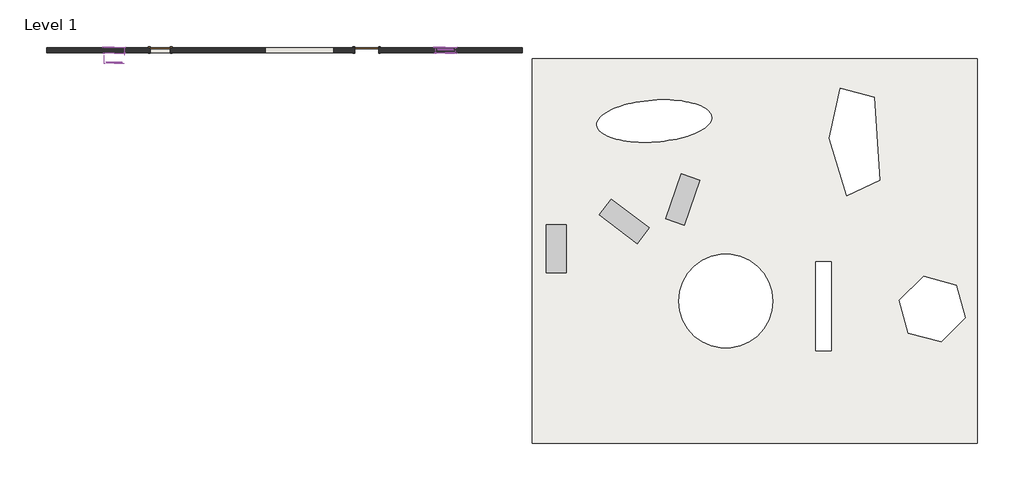
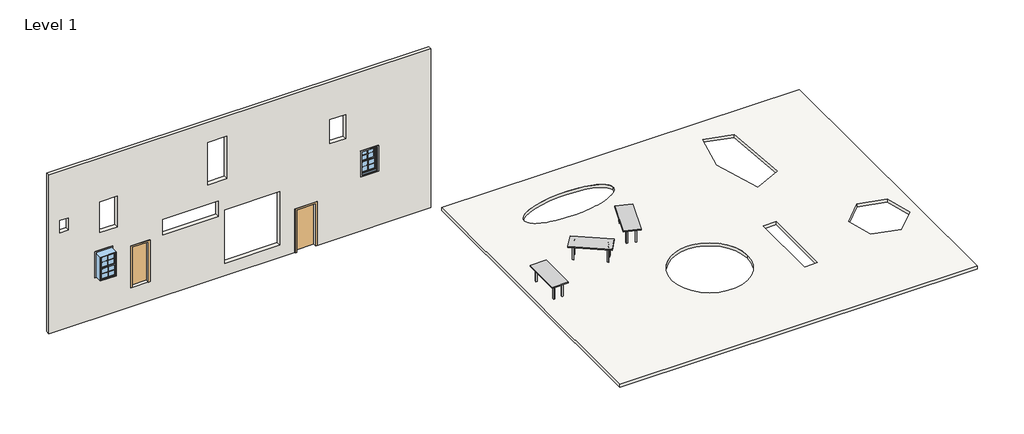
# One storey: 8 proxies, 3 furniture elements, 2 doors, 2 windows, 1 slab, 1 wall.
"""IFC4 building model written with IfcOpenShell, lengths in millimetres."""

import ifcopenshell
import ifcopenshell.guid

model = None  # the IFC model being written
_history = None  # IfcOwnerHistory: only IFC2X3 demands one
_inside = {}  # id of a spatial element -> (the spatial element, [elements in it])
_under = {}  # id of a project, library or spatial element -> (it, [spatial elements below it])
_declared = {}  # id of a project -> (the project, [libraries it declares])
_typed = {}  # id of a type object -> (the type object, [elements of that type])
_made_of = {}  # id of a material, layer set ... -> (it, [elements and type objects made of it])


def new_model(schema):
    """Start an empty IFC model of exactly this schema.

    Asked for "IFC4X3", IfcOpenShell would pick the latest addendum, in which some entities
    have other attributes; the version numbers below select the first issue.
    IFC2X3 requires an IfcOwnerHistory on every rooted entity: one is made here for all.
    """
    global model, _history
    if schema == "IFC4X3":
        model = ifcopenshell.file(schema_version=(4, 3, 0, 0))
    else:
        model = ifcopenshell.file(schema=schema)
    _inside.clear()
    _under.clear()
    _declared.clear()
    _typed.clear()
    _made_of.clear()
    _history = None
    if model.schema == "IFC2X3":
        org = make("IfcOrganization", Name="unknown")
        user = make(
            "IfcPersonAndOrganization",
            ThePerson=make("IfcPerson", FamilyName="unknown"),
            TheOrganization=org,
        )
        app = make(
            "IfcApplication",
            ApplicationDeveloper=org,
            Version="unknown",
            ApplicationFullName="unknown",
            ApplicationIdentifier="unknown",
        )
        _history = make(
            "IfcOwnerHistory",
            OwningUser=user,
            OwningApplication=app,
            ChangeAction="ADDED",
            CreationDate=0,
        )
    return model


def make(cls, **values):
    """One entity of the class cls with the attributes given. An attribute that is None is left unset."""
    return model.create_entity(
        cls, **{name: value for name, value in values.items() if value is not None}
    )


def rooted(cls, **values):
    """An entity with a GlobalId (a new one), such as an element, a storey or a relation."""
    return make(cls, GlobalId=ifcopenshell.guid.new(), OwnerHistory=_history, **values)


def si_unit(unit_type, name, prefix=None):
    """IfcSIUnit, for example si_unit("LENGTHUNIT", "METRE", prefix="MILLI")."""
    return make("IfcSIUnit", UnitType=unit_type, Prefix=prefix, Name=name)


def assignment(units):
    """IfcUnitAssignment: the units of a project."""
    return None if units is None else make("IfcUnitAssignment", Units=units)


def point(xyz):
    """IfcCartesianPoint."""
    return None if xyz is None else make("IfcCartesianPoint", Coordinates=xyz)


def direction(xyz):
    """IfcDirection."""
    return None if xyz is None else make("IfcDirection", DirectionRatios=xyz)


def frame(location, z_axis=None, x_axis=None):
    """IfcAxis2Placement3D, a coordinate frame: its origin and axes. An axis left out is left unset."""
    return make(
        "IfcAxis2Placement3D",
        Location=point(location),
        Axis=direction(z_axis),
        RefDirection=direction(x_axis),
    )


def origin():
    """The frame at (0, 0, 0) with its axes left unset."""
    return frame((0.0, 0.0, 0.0))


def origin_with_axes():
    """The frame at (0, 0, 0) with the z axis (0, 0, 1) and the x axis (1, 0, 0) written out."""
    return frame((0.0, 0.0, 0.0), z_axis=(0.0, 0.0, 1.0), x_axis=(1.0, 0.0, 0.0))


def place(relative_to, where):
    """IfcLocalPlacement: puts the frame where relative to a parent placement (None: the world)."""
    return make(
        "IfcLocalPlacement", PlacementRelTo=relative_to, RelativePlacement=where
    )


def context(
    kind, dimensions, precision=None, world=None, true_north=None, identifier=None
):
    """IfcGeometricRepresentationContext, for example the 3D "Model" context."""
    return make(
        "IfcGeometricRepresentationContext",
        ContextIdentifier=identifier,
        ContextType=kind,
        CoordinateSpaceDimension=dimensions,
        Precision=precision,
        WorldCoordinateSystem=world,
        TrueNorth=true_north,
    )


def project(units=None, contexts=None):
    """IfcProject with its units and contexts."""
    return rooted(
        "IfcProject",
        Name="project",
        RepresentationContexts=contexts,
        UnitsInContext=assignment(units),
    )


def spatial(cls, under=None, at=None, **own):
    """A site, building, storey or space (cls), placed at a placement, below another one or the project."""
    s = rooted(cls, ObjectPlacement=at, **own)
    if under is not None:
        _under.setdefault(under.id(), (under, []))[1].append(s)
    return s


def polyline(points):
    """IfcPolyline through the points."""
    return make("IfcPolyline", Points=[point(p) for p in points])


def circle_curve(where, radius):
    """IfcCircle in the frame where."""
    return make("IfcCircle", Position=where, Radius=radius)


def ellipse_curve(where, semi_axis1, semi_axis2):
    """IfcEllipse in the frame where."""
    return make(
        "IfcEllipse", Position=where, SemiAxis1=semi_axis1, SemiAxis2=semi_axis2
    )


def trimmed(basis, trim1, trim2, sense, master):
    """IfcTrimmedCurve: the piece of a basis curve between two trims."""
    return make(
        "IfcTrimmedCurve",
        BasisCurve=basis,
        Trim1=trim1,
        Trim2=trim2,
        SenseAgreement=sense,
        MasterRepresentation=master,
    )


def outline(outer, holes=None, kind="AREA"):
    """IfcArbitraryClosedProfileDef: a profile drawn as a closed curve; with holes, ...WithVoids."""
    if holes is None:
        return make("IfcArbitraryClosedProfileDef", ProfileType=kind, OuterCurve=outer)
    return make(
        "IfcArbitraryProfileDefWithVoids",
        ProfileType=kind,
        OuterCurve=outer,
        InnerCurves=holes,
    )


def extrude(swept, where, along, depth):
    """IfcExtrudedAreaSolid: the profile swept, set in the frame where, extruded along a direction by depth."""
    return make(
        "IfcExtrudedAreaSolid",
        SweptArea=swept,
        Position=where,
        ExtrudedDirection=direction(along),
        Depth=depth,
    )


def shape(context_of_items, identifier, shape_type, items):
    """IfcShapeRepresentation: the items that make up one representation, for example the "Body"."""
    return make(
        "IfcShapeRepresentation",
        ContextOfItems=context_of_items,
        RepresentationIdentifier=identifier,
        RepresentationType=shape_type,
        Items=items,
    )


def source(mapping_origin, context_of_items, identifier, shape_type, items):
    """IfcRepresentationMap: a shape defined once, which mapped items show again and again."""
    return make(
        "IfcRepresentationMap",
        MappingOrigin=mapping_origin,
        MappedRepresentation=shape(context_of_items, identifier, shape_type, items),
    )


def transform(
    local_origin,
    x_axis=None,
    y_axis=None,
    z_axis=None,
    scale=None,
    scale2=None,
    scale3=None,
    uniform=True,
):
    """IfcCartesianTransformationOperator3D, or its non-uniform kind. x_axis, y_axis, z_axis: its Axis1, 2, 3."""
    if uniform:
        return make(
            "IfcCartesianTransformationOperator3D",
            Axis1=direction(x_axis),
            Axis2=direction(y_axis),
            LocalOrigin=point(local_origin),
            Scale=scale,
            Axis3=direction(z_axis),
        )
    return make(
        "IfcCartesianTransformationOperator3DnonUniform",
        Axis1=direction(x_axis),
        Axis2=direction(y_axis),
        LocalOrigin=point(local_origin),
        Scale=scale,
        Axis3=direction(z_axis),
        Scale2=scale2,
        Scale3=scale3,
    )


def mapped(mapping_source, mapping_target):
    """IfcMappedItem: shows the shape of a source again, moved by a transform."""
    return make(
        "IfcMappedItem", MappingSource=mapping_source, MappingTarget=mapping_target
    )


def made_of(thing, what):
    """Note that an element or type object is made of a material, layer set ...; save() writes the relation."""
    if what is not None:
        _made_of.setdefault(what.id(), (what, []))[1].append(thing)
    return thing


def element(
    cls,
    number,
    at=None,
    inside=None,
    cuts=None,
    type_object=None,
    material=None,
    context=None,
    identifier="Body",
    shape_type=None,
    held_by="IfcProductDefinitionShape",
    body=None,
    shapes=None,
    **own,
):
    """One element of the class cls, such as IfcWall. Its Tag is "e" and its number.

    at: its placement. inside: the storey or other place that contains it. cuts: it is an
    opening in that element (IfcRelVoidsElement). A single representation is given by context,
    identifier, shape_type and body (its items); several are given by shapes. held_by: the class
    of the entity that holds the representations. save() writes the other relations.
    """
    e = rooted(cls, Tag="e%d" % number, ObjectPlacement=at, **own)
    if body is not None:
        shapes = [shape(context, identifier, shape_type, body)]
    if shapes is not None:
        e.Representation = make(held_by, Representations=shapes)
    if inside is not None:
        _inside.setdefault(inside.id(), (inside, []))[1].append(e)
    if cuts is not None:
        rooted(
            "IfcRelVoidsElement", RelatingBuildingElement=cuts, RelatedOpeningElement=e
        )
    if type_object is not None:
        _typed.setdefault(type_object.id(), (type_object, []))[1].append(e)
    return made_of(e, material)


def aggregate(whole, parts):
    """IfcRelAggregates: a whole, such as a stair, and the parts it consists of."""
    return rooted("IfcRelAggregates", RelatingObject=whole, RelatedObjects=parts)


def save(model, path):
    """Write the relations noted so far, then the file.

    IfcRelAggregates (storeys below a building ...), IfcRelContainedInSpatialStructure (elements
    in a storey), IfcRelDefinesByType, IfcRelAssociatesMaterial and IfcRelDeclares: one each for
    every whole, place, type object, material and project.
    """
    for whole, parts in _under.values():
        aggregate(whole, parts)
    for where, things in _inside.values():
        rooted(
            "IfcRelContainedInSpatialStructure",
            RelatedElements=things,
            RelatingStructure=where,
        )
    for kind, things in _typed.values():
        rooted("IfcRelDefinesByType", RelatedObjects=things, RelatingType=kind)
    for what, things in _made_of.values():
        rooted("IfcRelAssociatesMaterial", RelatedObjects=things, RelatingMaterial=what)
    for by, libraries in _declared.values():
        rooted("IfcRelDeclares", RelatingContext=by, RelatedDefinitions=libraries)
    model.write(path)


def plane_surface(at):
    """IfcPlane: the flat surface through the origin of the frame at, square to its z axis."""
    return make("IfcPlane", Position=at)


def revolved_surface(curve, axis_point, axis_direction):
    """IfcSurfaceOfRevolution: the curve turned about the line through axis_point along axis_direction."""
    return make(
        "IfcSurfaceOfRevolution",
        SweptCurve=make("IfcArbitraryOpenProfileDef", ProfileType="CURVE", Curve=curve),
        AxisPosition=make("IfcAxis1Placement", Location=point(axis_point), Axis=direction(axis_direction)),
    )


def extruded_surface(curve, direction_of_extrusion, depth):
    """IfcSurfaceOfLinearExtrusion: the curve pushed along a direction by depth."""
    return make(
        "IfcSurfaceOfLinearExtrusion",
        SweptCurve=make("IfcArbitraryOpenProfileDef", ProfileType="CURVE", Curve=curve),
        ExtrudedDirection=direction(direction_of_extrusion),
        Depth=depth,
    )


def advanced_brep(points, edges, surfaces, faces):
    """IfcAdvancedBrep: a solid bounded by faces that lie on surfaces and meet in shared edges.

    An edge is (start, end): straight between two places in points (the first is 0);
    or (start, end, curve); or (start, end, curve, False) where it runs against its curve.
    A face is (place in surfaces, loops), or (place, loops, False) where it looks against
    its surface's normal. A loop lists edges by number (the first is 1), with a minus sign
    where the edge is run from its end to its start. The first loop is the outer one.
    """
    corners = [point(p) for p in points]
    vertices = [make("IfcVertexPoint", VertexGeometry=c) for c in corners]
    made = []
    for start, end, *more in edges:
        made.append(
            make(
                "IfcEdgeCurve",
                EdgeStart=vertices[start],
                EdgeEnd=vertices[end],
                EdgeGeometry=more[0] if more else make("IfcPolyline", Points=[corners[start], corners[end]]),
                SameSense=more[1] if len(more) > 1 else True,
            )
        )
    hull = []
    for where, loops, *sense in faces:
        bounds = []
        for j, loop in enumerate(loops):
            ring = [make("IfcOrientedEdge", EdgeElement=made[abs(k) - 1], Orientation=k > 0) for k in loop]
            bounds.append(
                make(
                    "IfcFaceOuterBound" if j == 0 else "IfcFaceBound",
                    Bound=make("IfcEdgeLoop", EdgeList=ring),
                    Orientation=True,
                )
            )
        hull.append(make("IfcAdvancedFace", Bounds=bounds, FaceSurface=surfaces[where], SameSense=sense[0] if sense else True))
    return make("IfcAdvancedBrep", Outer=make("IfcClosedShell", CfsFaces=hull))


def m_muntin_pattern_2x2_m_muntin_pattern_2x2_aaec3afb(model_context):
    return source(origin(), model_context, "Body", "SweptSolid", [
        extrude(outline(polyline([(257.1375, -6.35), (257.1375, -298.8), (244.4375, -298.8), (244.4375, -6.35), (0.0, -6.35), (0.0, 6.35), (244.4375, 6.35), (244.4375, 298.8), (257.1375, 298.8), (257.1375, 6.35), (501.575, 6.35), (501.575, -6.35), (257.1375, -6.35)])), frame((0.0, 9.525, 0.0), z_axis=(0.0, 1.0, 0.0), x_axis=(0.0, 0.0, 1.0)), (0.0, 0.0, 1.0), 12.7),
        extrude(outline(polyline([(257.1375, -6.35), (257.1375, -298.8), (244.4375, -298.8), (244.4375, -6.35), (0.0, -6.35), (0.0, 6.35), (244.4375, 6.35), (244.4375, 298.8), (257.1375, 298.8), (257.1375, 6.35), (501.575, 6.35), (501.575, -6.35), (257.1375, -6.35)])), frame((0.0, -22.225, 0.0), z_axis=(0.0, 1.0, 0.0), x_axis=(0.0, 0.0, 1.0)), (0.0, 0.0, 1.0), 12.7),
    ])


def m_trim_window_exterior_flat_with_sill_e7ff6350(model_context):
    return source(origin(), model_context, "Body", "SweptSolid", [
        extrude(outline(polyline([(435.0, -1220.4323709), (435.0, -1280.4323709), (-435.0, -1280.4323709), (-435.0, -1220.4323709), (435.0, -1220.4323709)])), origin_with_axes(), (0.0, 0.0, 1.0), 19.05),
        extrude(outline(polyline([(-1230.0, 38.1), (-1202.4580645, 38.1), (-1200.0, 19.05), (-1200.0, 0.0), (-1220.4323709, 0.0), (-1220.4323709, 19.05), (-1230.0, 19.05), (-1230.0, 38.1)])), frame((-447.7, 0.0, 0.0), z_axis=(1.0, 0.0, 0.0), x_axis=(0.0, 1.0, 0.0)), (0.0, 0.0, 1.0), 895.4),
        extrude(outline(polyline([(-435.0, 60.0), (435.0, 60.0), (435.0, -1200.0), (375.0, -1200.0), (375.0, 0.0), (-375.0, 0.0), (-375.0, -1200.0), (-435.0, -1200.0), (-435.0, 60.0)])), origin_with_axes(), (0.0, 0.0, 1.0), 19.05),
    ])


def m_trim_window_interior_flat_picture_frame_31bd2320(model_context):
    return source(origin(), model_context, "Body", "SweptSolid", [
        extrude(outline(polyline([(422.3, 47.3), (422.3, -1247.3), (-422.3, -1247.3), (-422.3, 47.3), (422.3, 47.3)]), holes=[polyline([(362.3, -12.7), (-362.3, -12.7), (-362.3, -1187.3), (362.3, -1187.3), (362.3, -12.7)])]), origin_with_axes(), (0.0, 0.0, 1.0), 30.0),
    ])


def m_single_flush_0762_x_2032mm_0c256fab(model_context):
    return source(origin(), model_context, "Body", "SweptSolid", [
        extrude(outline(polyline([(2108.0, -457.0), (0.0, -457.0), (0.0, -381.0), (2032.0, -381.0), (2032.0, 381.0), (0.0, 381.0), (0.0, 457.0), (2108.0, 457.0), (2108.0, -457.0)])), frame((0.0, 100.0, 0.0), z_axis=(0.0, 1.0, 0.0), x_axis=(0.0, 0.0, 1.0)), (0.0, 0.0, 1.0), 25.0),
        extrude(outline(polyline([(2108.0, 457.0), (2108.0, -457.0), (0.0, -457.0), (0.0, -381.0), (2032.0, -381.0), (2032.0, 381.0), (0.0, 381.0), (0.0, 457.0), (2108.0, 457.0)])), frame((0.0, -125.0, 0.0), z_axis=(0.0, 1.0, 0.0), x_axis=(0.0, 0.0, 1.0)), (0.0, 0.0, 1.0), 25.0),
        extrude(outline(polyline([(381.0, 49.0), (-381.0, 49.0), (-381.0, 100.0), (381.0, 100.0), (381.0, 49.0)])), origin_with_axes(), (0.0, 0.0, 1.0), 2032.0),
    ])


def m_single_flush_0915_x_2134mm_727434cd(model_context):
    return source(origin(), model_context, "Body", "SweptSolid", [
        extrude(outline(polyline([(2210.0, -533.5), (0.0, -533.5), (0.0, -457.5), (2134.0, -457.5), (2134.0, 457.5), (0.0, 457.5), (0.0, 533.5), (2210.0, 533.5), (2210.0, -533.5)])), frame((0.0, -125.0, 0.0), z_axis=(0.0, 1.0, 0.0), x_axis=(0.0, 0.0, 1.0)), (0.0, 0.0, 1.0), 25.0),
        extrude(outline(polyline([(2210.0, 533.5), (2210.0, -533.5), (0.0, -533.5), (0.0, -457.5), (2134.0, -457.5), (2134.0, 457.5), (0.0, 457.5), (0.0, 533.5), (2210.0, 533.5)])), frame((0.0, 100.0, 0.0), z_axis=(0.0, 1.0, 0.0), x_axis=(0.0, 0.0, 1.0)), (0.0, 0.0, 1.0), 25.0),
        extrude(outline(polyline([(457.5, -49.0), (457.5, -100.0), (-457.5, -100.0), (-457.5, -49.0), (457.5, -49.0)])), origin_with_axes(), (0.0, 0.0, 1.0), 2134.0),
    ])


def m_table_rectangular_1830_x_0762mm_a0b3b7a0(model_context):
    return source(origin(), model_context, "Body", "SweptSolid", [
        extrude(outline(polyline([(699.1, 190.5), (699.1, 165.1), (-699.1, 165.1), (-699.1, 190.5), (699.1, 190.5)])), frame((0.0, 0.0, 609.6), z_axis=(0.0, 0.0, 1.0), x_axis=(1.0, 0.0, 0.0)), (0.0, 0.0, 1.0), 101.6),
        extrude(outline(polyline([(699.1, -190.5), (-699.1, -190.5), (-699.1, -165.1), (699.1, -165.1), (699.1, -190.5)])), frame((0.0, 0.0, 609.6), z_axis=(0.0, 0.0, 1.0), x_axis=(1.0, 0.0, 0.0)), (0.0, 0.0, 1.0), 101.6),
        extrude(outline(polyline([(-711.8, -165.1), (-737.2, -165.1), (-737.2, 165.1), (-711.8, 165.1), (-711.8, -165.1)])), frame((0.0, 0.0, 609.6), z_axis=(0.0, 0.0, 1.0), x_axis=(1.0, 0.0, 0.0)), (0.0, 0.0, 1.0), 101.6),
        extrude(outline(polyline([(711.8, -165.1), (711.8, 165.1), (737.2, 165.1), (737.2, -165.1), (711.8, -165.1)])), frame((0.0, 0.0, 609.6), z_axis=(0.0, 0.0, 1.0), x_axis=(1.0, 0.0, 0.0)), (0.0, 0.0, 1.0), 101.6),
        extrude(outline(polyline([(915.0, 381.0), (915.0, -381.0), (-915.0, -381.0), (-915.0, 381.0), (915.0, 381.0)])), frame((0.0, 0.0, 711.2), z_axis=(0.0, 0.0, 1.0), x_axis=(1.0, 0.0, 0.0)), (0.0, 0.0, 1.0), 50.8),
        extrude(outline(polyline([(-699.1, 228.6), (-699.1, 165.1), (-762.6, 165.1), (-762.6, 228.6), (-699.1, 228.6)])), origin_with_axes(), (0.0, 0.0, 1.0), 711.2),
        extrude(outline(polyline([(699.1, 228.6), (762.6, 228.6), (762.6, 165.1), (699.1, 165.1), (699.1, 228.6)])), origin_with_axes(), (0.0, 0.0, 1.0), 711.2),
        extrude(outline(polyline([(-699.1, -228.6), (-762.6, -228.6), (-762.6, -165.1), (-699.1, -165.1), (-699.1, -228.6)])), origin_with_axes(), (0.0, 0.0, 1.0), 711.2),
        extrude(outline(polyline([(699.1, -228.6), (699.1, -165.1), (762.6, -165.1), (762.6, -228.6), (699.1, -228.6)])), origin_with_axes(), (0.0, 0.0, 1.0), 711.2),
    ])


def m_window_double_hung_750_x_1200mm_e21ea802(model_context):
    return source(origin(), model_context, "Body", "SweptSolid", [
        extrude(outline(polyline([(298.8, -469.85), (298.8, -476.2), (-298.8, -476.2), (-298.8, -469.85), (298.8, -469.85)])), frame((0.0, 0.0, 990.6), z_axis=(0.0, 0.0, 1.0), x_axis=(1.0, 0.0, 0.0)), (0.0, 0.0, 1.0), 501.575),
        extrude(outline(polyline([(-298.8, -482.55), (298.8, -482.55), (298.8, -488.9), (-298.8, -488.9), (-298.8, -482.55)])), frame((0.0, 0.0, 990.6), z_axis=(0.0, 0.0, 1.0), x_axis=(1.0, 0.0, 0.0)), (0.0, 0.0, 1.0), 501.575),
        extrude(outline(polyline([(298.8, -425.4), (298.8, -431.75), (-298.8, -431.75), (-298.8, -425.4), (298.8, -425.4)])), frame((0.0, 0.0, 1536.625), z_axis=(0.0, 0.0, 1.0), x_axis=(1.0, 0.0, 0.0)), (0.0, 0.0, 1.0), 501.575),
        extrude(outline(polyline([(-298.8, -438.1), (298.8, -438.1), (298.8, -444.45), (-298.8, -444.45), (-298.8, -438.1)])), frame((0.0, 0.0, 1536.625), z_axis=(0.0, 0.0, 1.0), x_axis=(1.0, 0.0, 0.0)), (0.0, 0.0, 1.0), 501.575),
        extrude(outline(polyline([(1536.625, -343.25), (946.15, -343.25), (946.15, 343.25), (1536.625, 343.25), (1536.625, -343.25)]), holes=[polyline([(1492.175, 298.8), (990.6, 298.8), (990.6, -298.8), (1492.175, -298.8), (1492.175, 298.8)])]), frame((0.0, -501.6, 0.0), z_axis=(0.0, 1.0, 0.0), x_axis=(0.0, 0.0, 1.0)), (0.0, 0.0, 1.0), 44.45),
        extrude(outline(polyline([(2082.65, -343.25), (1492.175, -343.25), (1492.175, 343.25), (2082.65, 343.25), (2082.65, -343.25)]), holes=[polyline([(2038.2, 298.8), (1536.625, 298.8), (1536.625, -298.8), (2038.2, -298.8), (2038.2, 298.8)])]), frame((0.0, -457.15, 0.0), z_axis=(0.0, 1.0, 0.0), x_axis=(0.0, 0.0, 1.0)), (0.0, 0.0, 1.0), 44.45),
        extrude(outline(polyline([(2114.4, -375.0), (914.4, -375.0), (914.4, 375.0), (2114.4, 375.0), (2114.4, -375.0)]), holes=[polyline([(2082.65, 343.25), (946.15, 343.25), (946.15, -343.25), (2082.65, -343.25), (2082.65, 343.25)])]), frame((0.0, -514.3, 0.0), z_axis=(0.0, 1.0, 0.0), x_axis=(0.0, 0.0, 1.0)), (0.0, 0.0, 1.0), 633.35),
    ])


def m_window_double_hung_750_x_1200mm_41070976(model_context):
    return source(origin(), model_context, "Body", "SweptSolid", [
        extrude(outline(polyline([(298.8, 30.15), (298.8, 23.8), (-298.8, 23.8), (-298.8, 30.15), (298.8, 30.15)])), frame((0.0, 0.0, 990.6), z_axis=(0.0, 0.0, 1.0), x_axis=(1.0, 0.0, 0.0)), (0.0, 0.0, 1.0), 501.575),
        extrude(outline(polyline([(-298.8, 17.45), (298.8, 17.45), (298.8, 11.1), (-298.8, 11.1), (-298.8, 17.45)])), frame((0.0, 0.0, 990.6), z_axis=(0.0, 0.0, 1.0), x_axis=(1.0, 0.0, 0.0)), (0.0, 0.0, 1.0), 501.575),
        extrude(outline(polyline([(298.8, 74.6), (298.8, 68.25), (-298.8, 68.25), (-298.8, 74.6), (298.8, 74.6)])), frame((0.0, 0.0, 1536.625), z_axis=(0.0, 0.0, 1.0), x_axis=(1.0, 0.0, 0.0)), (0.0, 0.0, 1.0), 501.575),
        extrude(outline(polyline([(-298.8, 61.9), (298.8, 61.9), (298.8, 55.55), (-298.8, 55.55), (-298.8, 61.9)])), frame((0.0, 0.0, 1536.625), z_axis=(0.0, 0.0, 1.0), x_axis=(1.0, 0.0, 0.0)), (0.0, 0.0, 1.0), 501.575),
        extrude(outline(polyline([(1536.625, -343.25), (946.15, -343.25), (946.15, 343.25), (1536.625, 343.25), (1536.625, -343.25)]), holes=[polyline([(1492.175, 298.8), (990.6, 298.8), (990.6, -298.8), (1492.175, -298.8), (1492.175, 298.8)])]), frame((0.0, -1.6, 0.0), z_axis=(0.0, 1.0, 0.0), x_axis=(0.0, 0.0, 1.0)), (0.0, 0.0, 1.0), 44.45),
        extrude(outline(polyline([(2082.65, -343.25), (1492.175, -343.25), (1492.175, 343.25), (2082.65, 343.25), (2082.65, -343.25)]), holes=[polyline([(2038.2, 298.8), (1536.625, 298.8), (1536.625, -298.8), (2038.2, -298.8), (2038.2, 298.8)])]), frame((0.0, 42.85, 0.0), z_axis=(0.0, 1.0, 0.0), x_axis=(0.0, 0.0, 1.0)), (0.0, 0.0, 1.0), 44.45),
        extrude(outline(polyline([(2114.4, -375.0), (914.4, -375.0), (914.4, 375.0), (2114.4, 375.0), (2114.4, -375.0)]), holes=[polyline([(2082.65, 343.25), (946.15, 343.25), (946.15, -343.25), (2082.65, -343.25), (2082.65, 343.25)])]), frame((0.0, -14.3, 0.0), z_axis=(0.0, 1.0, 0.0), x_axis=(0.0, 0.0, 1.0)), (0.0, 0.0, 1.0), 133.35),
        extrude(outline(polyline([(2114.4, 375.0), (2114.4, -375.0), (914.4, -375.0), (914.4, 375.0), (2114.4, 375.0)]), holes=[polyline([(2095.35, 355.95), (933.45, 355.95), (933.45, -355.95), (2095.35, -355.95), (2095.35, 355.95)])]), frame((0.0, -100.0, 0.0), z_axis=(0.0, 1.0, 0.0), x_axis=(0.0, 0.0, 1.0)), (0.0, 0.0, 1.0), 85.7),
    ])


model = new_model("IFC4")

# Units and contexts
model_context = context("Model", 3, world=origin())
ifc_project = project(units=[si_unit("LENGTHUNIT", "METRE", prefix="MILLI")], contexts=[model_context])

# Site, building, storey
site = spatial("IfcSite", under=ifc_project)
building = spatial("IfcBuilding", under=site)
storey = spatial("IfcBuildingStorey", under=building, Name="Level 1", Elevation=0.0)

# Proxies
placement = place(None, origin())
m_muntin_pattern_2x2_m_muntin_pattern_2x2_shape = m_muntin_pattern_2x2_m_muntin_pattern_2x2_aaec3afb(model_context)
element("IfcBuildingElementProxy", 1, Name="M_Muntin Pattern_2x2 : M_Muntin Pattern_2x2", ObjectType="M_Muntin Pattern_2x2 : M_Muntin Pattern_2x2", at=placement, inside=storey, context=model_context, shape_type="MappedRepresentation", body=[
    mapped(m_muntin_pattern_2x2_m_muntin_pattern_2x2_shape, transform((-13755.2543844, 2099.5505832, 3404.9440493), x_axis=(1.0, 0.0, 0.0), y_axis=(0.0, 1.0, 0.0), z_axis=(0.0, 0.0, 1.0))),
])
element("IfcBuildingElementProxy", 2, Name="M_Muntin Pattern_2x2 : M_Muntin Pattern_2x2", ObjectType="M_Muntin Pattern_2x2 : M_Muntin Pattern_2x2", at=placement, inside=storey, context=model_context, shape_type="MappedRepresentation", body=[
    mapped(m_muntin_pattern_2x2_m_muntin_pattern_2x2_shape, transform((-13755.2543844, 2055.1005832, 2858.9190493), x_axis=(1.0, 0.0, 0.0), y_axis=(0.0, 1.0, 0.0), z_axis=(0.0, 0.0, 1.0))),
])
element("IfcBuildingElementProxy", 3, Name="M_Muntin Pattern_2x2 : M_Muntin Pattern_2x2", ObjectType="M_Muntin Pattern_2x2 : M_Muntin Pattern_2x2", at=placement, inside=storey, context=model_context, shape_type="MappedRepresentation", body=[
    mapped(m_muntin_pattern_2x2_m_muntin_pattern_2x2_shape, transform((-26427.6862127, 1599.5505832, 2762.3712435), x_axis=(1.0, 0.0, 0.0), y_axis=(0.0, 1.0, 0.0), z_axis=(0.0, 0.0, 1.0))),
])
element("IfcBuildingElementProxy", 4, Name="M_Muntin Pattern_2x2 : M_Muntin Pattern_2x2", ObjectType="M_Muntin Pattern_2x2 : M_Muntin Pattern_2x2", at=placement, inside=storey, context=model_context, shape_type="MappedRepresentation", body=[
    mapped(m_muntin_pattern_2x2_m_muntin_pattern_2x2_shape, transform((-26427.6862127, 1555.1005832, 2216.3462435), x_axis=(1.0, 0.0, 0.0), y_axis=(0.0, 1.0, 0.0), z_axis=(0.0, 0.0, 1.0))),
])
m_trim_window_exterior_flat_with_sill_shape = m_trim_window_exterior_flat_with_sill_e7ff6350(model_context)
element("IfcBuildingElementProxy", 5, Name="M_Trim-Window-Exterior-Flat : with Sill", ObjectType="M_Trim-Window-Exterior-Flat : with Sill", at=placement, inside=storey, context=model_context, shape_type="MappedRepresentation", body=[
    mapped(m_trim_window_exterior_flat_with_sill_shape, transform((-13755.2543844, 2134.4755832, 3982.7190493), x_axis=(-1.0, 0.0, 0.0), y_axis=(0.0, 0.0, 1.0), z_axis=(0.0, 1.0, 0.0))),
])
element("IfcBuildingElementProxy", 6, Name="M_Trim-Window-Exterior-Flat : with Sill", ObjectType="M_Trim-Window-Exterior-Flat : with Sill", at=placement, inside=storey, context=model_context, shape_type="MappedRepresentation", body=[
    mapped(m_trim_window_exterior_flat_with_sill_shape, transform((-26427.6862127, 2134.4755832, 3340.1462435), x_axis=(-1.0, 0.0, 0.0), y_axis=(0.0, 0.0, 1.0), z_axis=(0.0, 1.0, 0.0))),
])
m_trim_window_interior_flat_picture_frame_shape = m_trim_window_interior_flat_picture_frame_31bd2320(model_context)
element("IfcBuildingElementProxy", 7, Name="M_Trim-Window-Interior-Flat : Picture Frame", ObjectType="M_Trim-Window-Interior-Flat : Picture Frame", at=placement, inside=storey, context=model_context, shape_type="MappedRepresentation", body=[
    mapped(m_trim_window_interior_flat_picture_frame_shape, transform((-13755.2543844, 1934.4755832, 3982.7190493), x_axis=(1.0, 0.0, 0.0), y_axis=(0.0, 0.0, 1.0), z_axis=(0.0, -1.0, 0.0))),
])
element("IfcBuildingElementProxy", 8, Name="M_Trim-Window-Interior-Flat : Picture Frame", ObjectType="M_Trim-Window-Interior-Flat : Picture Frame", at=placement, inside=storey, context=model_context, shape_type="MappedRepresentation", body=[
    mapped(m_trim_window_interior_flat_picture_frame_shape, transform((-26427.6862127, 1934.4755832, 3340.1462435), x_axis=(1.0, 0.0, 0.0), y_axis=(0.0, 0.0, 1.0), z_axis=(0.0, -1.0, 0.0))),
])

# Doors
m_single_flush_0762_x_2032mm_shape = m_single_flush_0762_x_2032mm_0c256fab(model_context)
element("IfcDoor", 9, ObjectType="M_Single-Flush : 0762 x 2032mm", at=placement, inside=storey, context=model_context, shape_type="MappedRepresentation", body=[
    mapped(m_single_flush_0762_x_2032mm_shape, transform((-24671.6862127, 2034.4755832, 968.0), x_axis=(1.0, 0.0, 0.0), y_axis=(0.0, 1.0, 0.0), z_axis=(0.0, 0.0, 1.0))),
])
m_single_flush_0915_x_2134mm_shape = m_single_flush_0915_x_2134mm_727434cd(model_context)
element("IfcDoor", 10, ObjectType="M_Single-Flush : 0915 x 2134mm", at=placement, inside=storey, context=model_context, shape_type="MappedRepresentation", body=[
    mapped(m_single_flush_0915_x_2134mm_shape, transform((-16774.8897659, 2034.4755832, 0.0), x_axis=(-1.0, 0.0, 0.0), y_axis=(0.0, -1.0, 0.0), z_axis=(0.0, 0.0, 1.0))),
])

# Furniture
m_table_rectangular_1830_x_0762mm_shape = m_table_rectangular_1830_x_0762mm_a0b3b7a0(model_context)
element("IfcFurniture", 11, ObjectType="M_Table-Rectangular : 1830 x 0762mm", at=placement, inside=storey, context=model_context, shape_type="MappedRepresentation", body=[
    mapped(m_table_rectangular_1830_x_0762mm_shape, transform((-4676.3852744, -3681.7142207, 0.0), x_axis=(-0.32556815445715137, -0.9455185755993186, 0.0), y_axis=(0.9455185755993186, -0.32556815445715137, 0.0), z_axis=(0.0, 0.0, 1.0))),
])
element("IfcFurniture", 12, ObjectType="M_Table-Rectangular : 1830 x 0762mm", at=placement, inside=storey, context=model_context, shape_type="MappedRepresentation", body=[
    mapped(m_table_rectangular_1830_x_0762mm_shape, transform((-6912.0232604, -4514.409007, 0.0), x_axis=(0.7986355100472892, -0.601815023152053, 0.0), y_axis=(0.601815023152053, 0.7986355100472892, 0.0), z_axis=(0.0, 0.0, 1.0))),
])
element("IfcFurniture", 13, ObjectType="M_Table-Rectangular : 1830 x 0762mm", at=placement, inside=storey, context=model_context, shape_type="MappedRepresentation", body=[
    mapped(m_table_rectangular_1830_x_0762mm_shape, transform((-9517.3897659, -5565.5244168, 0.0), x_axis=(0.0, 1.0, 0.0), y_axis=(-1.0, 0.0, 0.0), z_axis=(0.0, 0.0, 1.0))),
])

# Slab
element("IfcSlab", 14, ObjectType="Generic 150mm", at=placement, inside=storey, context=model_context, shape_type="AdvancedBrep", body=[
    advanced_brep(
    [(-10438.0920872, 1704.9536342, -150.0), (6597.1361468, 1704.9536342, -150.0), (6597.1361468, -12995.0463658, -150.0), (-10438.0920872, -12995.0463658, -150.0), (402.6850474, -6063.7932352, -150.0), (402.6850474, -9463.7932352, -150.0), (1002.6850474, -9463.7932352, -150.0), (1002.6850474, -6063.7932352, -150.0), (-1226.5132944, -7566.8871411, -150.0), (-4826.5132944, -7566.8871411, -150.0), (3950.2905395, -8793.2666419, -150.0), (5205.9941136, -9129.7314005, -150.0), (6125.2329292, -8210.492585, -150.0), (5788.7681706, -6954.7890108, -150.0), (4533.0645964, -6618.3242522, -150.0), (3613.8257808, -7537.5630677, -150.0), (2640.3105602, 236.4658339, -150.0), (1342.8691088, 584.1142231, -150.0), (924.6812259, -1326.1660948, -150.0), (1597.1361468, -3525.6670335, -150.0), (2862.1361468, -2935.7878459, -150.0), (-3571.6563241, -523.7317463, -150.0), (-7960.9381452, -830.6602307, -150.0), (6597.1361468, 1704.9536342, 0.0), (-10438.0920872, 1704.9536342, 0.0), (-10438.0920872, -12995.0463658, 0.0), (6597.1361468, -12995.0463658, 0.0), (402.6850474, -9463.7932352, 0.0), (402.6850474, -6063.7932352, 0.0), (1002.6850474, -6063.7932352, 0.0), (1002.6850474, -9463.7932352, 0.0), (-4826.5132944, -7566.8871411, 0.0), (-1226.5132944, -7566.8871411, 0.0), (5205.9941136, -9129.7314005, 0.0), (3950.2905395, -8793.2666419, 0.0), (3613.8257808, -7537.5630677, 0.0), (4533.0645964, -6618.3242522, 0.0), (5788.7681706, -6954.7890108, 0.0), (6125.2329292, -8210.492585, 0.0), (1342.8691088, 584.1142231, 0.0), (2640.3105602, 236.4658339, 0.0), (2862.1361468, -2935.7878459, 0.0), (1597.1361468, -3525.6670335, 0.0), (924.6812259, -1326.1660948, 0.0), (-7960.9381452, -830.6602307, 0.0), (-3571.6563241, -523.7317463, 0.0)],
    [
        (0, 1),
        (1, 2),
        (2, 3),
        (3, 0),
        (4, 5),
        (5, 6),
        (6, 7),
        (7, 4),
        (8, 9, circle_curve(frame((-3026.5132944, -7566.8871411, -150.0), z_axis=(0.0, 0.0, 1.0), x_axis=(-1.0, 0.0, 0.0)), 1800.0)),
        (9, 8, circle_curve(frame((-3026.5132944, -7566.8871411, -150.0), z_axis=(0.0, 0.0, 1.0), x_axis=(-1.0, 0.0, 0.0)), 1800.0)),
        (10, 11),
        (11, 12),
        (12, 13),
        (13, 14),
        (14, 15),
        (15, 10),
        (16, 17),
        (17, 18),
        (18, 19),
        (19, 20),
        (20, 16),
        (21, 22, ellipse_curve(frame((-5766.2972347, -677.1959885, -150.0), z_axis=(0.0, 0.0, 1.0), x_axis=(-0.9975640502598249, -0.06975647374411696, 0.0)), 2200.0, 800.0)),
        (22, 21, ellipse_curve(frame((-5766.2972347, -677.1959885, -150.0), z_axis=(0.0, 0.0, 1.0), x_axis=(-0.9975640502598249, -0.06975647374411696, 0.0)), 2200.0, 800.0)),
        (23, 24),
        (24, 25),
        (25, 26),
        (26, 23),
        (27, 28),
        (28, 29),
        (29, 30),
        (30, 27),
        (31, 32, circle_curve(frame((-3026.5132944, -7566.8871411, 0.0), z_axis=(0.0, 0.0, -1.0), x_axis=(-1.0, 0.0, 0.0)), 1800.0)),
        (32, 31, circle_curve(frame((-3026.5132944, -7566.8871411, 0.0), z_axis=(0.0, 0.0, -1.0), x_axis=(-1.0, 0.0, 0.0)), 1800.0)),
        (33, 34),
        (34, 35),
        (35, 36),
        (36, 37),
        (37, 38),
        (38, 33),
        (39, 40),
        (40, 41),
        (41, 42),
        (42, 43),
        (43, 39),
        (44, 45, ellipse_curve(frame((-5766.2972347, -677.1959885, 0.0), z_axis=(0.0, 0.0, -1.0), x_axis=(-0.9975640502598249, -0.06975647374411696, 0.0)), 2200.0, 800.0)),
        (45, 44, ellipse_curve(frame((-5766.2972347, -677.1959885, 0.0), z_axis=(0.0, 0.0, -1.0), x_axis=(-0.9975640502598249, -0.06975647374411696, 0.0)), 2200.0, 800.0)),
        (0, 24),
        (23, 1),
        (26, 2),
        (25, 3),
        (4, 28),
        (27, 5),
        (30, 6),
        (29, 7),
        (8, 32),
        (31, 9),
        (10, 34),
        (33, 11),
        (38, 12),
        (37, 13),
        (36, 14),
        (35, 15),
        (16, 40),
        (39, 17),
        (18, 43),
        (42, 19),
        (41, 20),
        (21, 45),
        (44, 22),
    ],
    [
        plane_surface(frame((5561.9079128, 1704.9536342, -150.0), z_axis=(0.0, 0.0, -1.0), x_axis=(1.0, 0.0, 0.0))),
        plane_surface(frame((5561.9079128, 1704.9536342, 0.0), z_axis=(0.0, 0.0, 1.0), x_axis=(-1.0, 0.0, 0.0))),
        plane_surface(frame((-10438.0920872, 1704.9536342, -150.0), z_axis=(0.0, 1.0, 0.0), x_axis=(0.0, 0.0, 1.0))),
        plane_surface(frame((6597.1361468, 1704.9536342, -150.0), z_axis=(1.0, 0.0, 0.0), x_axis=(0.0, 0.0, 1.0))),
        plane_surface(frame((6597.1361468, -12995.0463658, -150.0), z_axis=(0.0, -1.0, 0.0), x_axis=(0.0, 0.0, 1.0))),
        plane_surface(frame((-10438.0920872, -12995.0463658, -150.0), z_axis=(-1.0, 0.0, 0.0), x_axis=(0.0, 0.0, 1.0))),
        plane_surface(frame((402.6850474, -6063.7932352, 754.8), z_axis=(1.0, 0.0, 0.0), x_axis=(0.0, 0.0, -1.0))),
        plane_surface(frame((402.6850474, -9463.7932352, 754.8), z_axis=(0.0, 1.0, 0.0), x_axis=(0.0, 0.0, -1.0))),
        plane_surface(frame((1002.6850474, -9463.7932352, 754.8), z_axis=(-1.0, 0.0, 0.0), x_axis=(0.0, 0.0, -1.0))),
        plane_surface(frame((1002.6850474, -6063.7932352, 754.8), z_axis=(0.0, -1.0, 0.0), x_axis=(0.0, 0.0, -1.0))),
        revolved_surface(polyline([(-4826.5132944, -7566.8871411, 0.0), (-4826.5132944, -7566.8871411, -150.0)]), (-3026.5132944, -7566.8871411, -454.8), (0.0, 0.0, 1.0)),
        plane_surface(frame((3950.2905395, -8793.2666419, 754.8), z_axis=(0.2588190451025399, 0.9659258262890632, 0.0), x_axis=(0.0, 0.0, -1.0))),
        plane_surface(frame((5205.9941136, -9129.7314005, 754.8), z_axis=(-0.7071067811865333, 0.7071067811865619, 0.0), x_axis=(0.0, 0.0, -1.0))),
        plane_surface(frame((6125.2329292, -8210.492585, 754.8), z_axis=(-0.9659258262890744, -0.2588190451024985, 0.0), x_axis=(0.0, 0.0, -1.0))),
        plane_surface(frame((5788.7681706, -6954.7890108, 754.8), z_axis=(-0.25881904510254333, -0.9659258262890623, 0.0), x_axis=(0.0, 0.0, -1.0))),
        plane_surface(frame((4533.0645964, -6618.3242522, 754.8), z_axis=(0.7071067811865306, -0.7071067811865644, 0.0), x_axis=(0.0, 0.0, -1.0))),
        plane_surface(frame((3613.8257808, -7537.5630677, 754.8), z_axis=(0.965925826289073, 0.2588190451025034, 0.0), x_axis=(0.0, 0.0, -1.0))),
        plane_surface(frame((2640.3105602, 236.4658339, -150.0), z_axis=(-0.25881904510253306, -0.9659258262890651, 0.0), x_axis=(0.0, 0.0, 1.0))),
        plane_surface(frame((924.6812259, -1326.1660948, -150.0), z_axis=(0.9563047559630387, 0.29237170472272644, 0.0), x_axis=(0.0, 0.0, 1.0))),
        plane_surface(frame((1597.1361468, -3525.6670335, -150.0), z_axis=(-0.42261826174069067, 0.9063077870366542, 0.0), x_axis=(0.0, 0.0, 1.0))),
        plane_surface(frame((2862.1361468, -2935.7878459, -150.0), z_axis=(-0.997564050259825, -0.06975647374411523, 0.0), x_axis=(0.0, 0.0, 1.0))),
        plane_surface(frame((1342.8691088, 584.1142231, -150.0), z_axis=(0.9768664776736946, -0.21385014565669358, 0.0), x_axis=(0.0, 0.0, 1.0))),
        extruded_surface(trimmed(ellipse_curve(frame((-5766.2972347, -677.1959885, 150.0), z_axis=(0.0, 0.0, 1.0), x_axis=(-0.9975640502598249, -0.06975647374411696, 0.0)), 2200.0, 800.0), [point((-3571.6563241, -523.7317463, 150.0))], [point((-7960.9381452, -830.6602307, 150.0))], True, "CARTESIAN"), (0.0, 0.0, -150.0), 150.0),
        extruded_surface(trimmed(ellipse_curve(frame((-5766.2972347, -677.1959885, 150.0), z_axis=(0.0, 0.0, 1.0), x_axis=(-0.9975640502598249, -0.06975647374411696, 0.0)), 2200.0, 800.0), [point((-7960.9381452, -830.6602307, 150.0))], [point((-3571.6563241, -523.7317463, 150.0))], True, "CARTESIAN"), (0.0, 0.0, -150.0), 150.0),
    ],
    [
        (0, [[1, 2, 3, 4], [5, 6, 7, 8], [9, 10], [11, 12, 13, 14, 15, 16], [17, 18, 19, 20, 21], [22, 23]]),
        (1, [[24, 25, 26, 27], [28, 29, 30, 31], [32, 33], [34, 35, 36, 37, 38, 39], [40, 41, 42, 43, 44], [45, 46]]),
        (2, [[-1, 47, -24, 48]]),
        (3, [[-2, -48, -27, 49]]),
        (4, [[-3, -49, -26, 50]]),
        (5, [[-4, -50, -25, -47]]),
        (6, [[51, -28, 52, -5]]),
        (7, [[-52, -31, 53, -6]]),
        (8, [[-53, -30, 54, -7]]),
        (9, [[-51, -8, -54, -29]]),
        (10, [[55, -32, 56, -9]]),
        (10, [[-55, -10, -56, -33]]),
        (11, [[57, -34, 58, -11]]),
        (12, [[-58, -39, 59, -12]]),
        (13, [[-59, -38, 60, -13]]),
        (14, [[-60, -37, 61, -14]]),
        (15, [[-61, -36, 62, -15]]),
        (16, [[-57, -16, -62, -35]]),
        (17, [[-17, 63, -40, 64]]),
        (18, [[-19, 65, -43, 66]]),
        (19, [[-20, -66, -42, 67]]),
        (20, [[-21, -67, -41, -63]]),
        (21, [[-18, -64, -44, -65]]),
        (22, [[-22, 68, -45, 69]]),
        (23, [[-23, -69, -46, -68]]),
    ],
),
])

# Wall
element("IfcWall", 15, ObjectType="Generic - 200mm", at=placement, inside=storey, context=model_context, shape_type="SweptSolid", body=[
    extrude(outline(polyline([(8000.0, -29017.3897659), (0.0, -29017.3897659), (0.0, -17232.3897659), (2134.0, -17232.3897659), (2134.0, -16317.3897659), (0.0, -16317.3897659), (0.0, -10817.3897659), (8000.0, -10817.3897659), (8000.0, -29017.3897659)]), holes=[polyline([(968.0, -25052.6862127), (3000.0, -25052.6862127), (3000.0, -24290.6862127), (968.0, -24290.6862127), (968.0, -25052.6862127)]), polyline([(4915.0, -28496.5284847), (5525.0, -28496.5284847), (5525.0, -28090.5284847), (4915.0, -28090.5284847), (4915.0, -28496.5284847)]), polyline([(2140.1462435, -26802.6862127), (3340.1462435, -26802.6862127), (3340.1462435, -26052.6862127), (2140.1462435, -26052.6862127), (2140.1462435, -26802.6862127)]), polyline([(2782.7190493, -14130.2543844), (3982.7190493, -14130.2543844), (3982.7190493, -13380.2543844), (2782.7190493, -13380.2543844), (2782.7190493, -14130.2543844)]), polyline([(4914.4, -15639.9853759), (6114.4, -15639.9853759), (6114.4, -14889.9853759), (4914.4, -14889.9853759), (4914.4, -15639.9853759)]), polyline([(4866.0, -20539.9853759), (4866.0, -21454.9853759), (7000.0, -21454.9853759), (7000.0, -20539.9853759), (4866.0, -20539.9853759)]), polyline([(3328.9271244, -20644.8897659), (3328.9271244, -18024.3599995), (634.0, -18024.3599995), (634.0, -20644.8897659), (3328.9271244, -20644.8897659)]), polyline([(3873.453269, -23605.3752389), (3873.453269, -20944.8897659), (3100.0, -20944.8897659), (3100.0, -23605.3752389), (3873.453269, -23605.3752389)]), polyline([(5800.0, -26593.5284847), (5800.0, -25757.3810809), (4260.1064286, -25757.3810809), (4260.1064286, -26593.5284847), (5800.0, -26593.5284847)])]), frame((0.0, 1934.4755832, 0.0), z_axis=(0.0, 1.0, 0.0), x_axis=(0.0, 0.0, 1.0)), (0.0, 0.0, 1.0), 200.0),
])

# Windows
m_window_double_hung_750_x_1200mm_shape = m_window_double_hung_750_x_1200mm_e21ea802(model_context)
element("IfcWindow", 16, ObjectType="M_Window-Double-Hung : 750 x 1200mm", at=placement, inside=storey, context=model_context, shape_type="MappedRepresentation", body=[
    mapped(m_window_double_hung_750_x_1200mm_shape, transform((-26427.6862127, 2034.4755832, 1225.7462435), x_axis=(1.0, 0.0, 0.0), y_axis=(0.0, 1.0, 0.0), z_axis=(0.0, 0.0, 1.0))),
])
m_window_double_hung_750_x_1200mm_2_shape = m_window_double_hung_750_x_1200mm_41070976(model_context)
element("IfcWindow", 17, ObjectType="M_Window-Double-Hung : 750 x 1200mm", at=placement, inside=storey, context=model_context, shape_type="MappedRepresentation", body=[
    mapped(m_window_double_hung_750_x_1200mm_2_shape, transform((-13755.2543844, 2034.4755832, 1868.3190493), x_axis=(1.0, 0.0, 0.0), y_axis=(0.0, 1.0, 0.0), z_axis=(0.0, 0.0, 1.0))),
])

save(model, "model.ifc")

# Revit data of these elements
# Project information
#   Project Issue Date = "Issue Date"
#   Project Status = "Project Status"
#   Client Name = "Owner"
#   Project Address = "Enter address here"
#   Project Name = "Project Name"
#   Project Number = "0001"
# Type "M_Muntin Pattern_2x2 : M_Muntin Pattern_2x2"
#   Width [instance default] = 1200 mm
#   Thickness = 12.7 mm
#   Height [instance default] = 1200 mm
#   Distance = 19.05 mm
#   Interior Material [instance default] = none
#   Exterior Material [instance default] = none
#   Default Elevation = 0
# Type "M_Trim-Window-Exterior-Flat : with Sill"
#   Trim Width = 60 mm
#   Trim Thickness_Picture Frame = 30 mm
#   Trim Thickness_with Sill = 19.05 mm
#   Sill Thickness = 30 mm
#   Opening Width [instance default] = 600 mm
#   Opening Height [instance default] = 900 mm
#   Default Elevation = 1200 mm
#   Sill = yes
#   Picture Frame = no
#   Trim Material [instance default] = none
# Type "M_Trim-Window-Interior-Flat : Picture Frame"
#   Trim Thickness_Picture Frame = 30 mm
#   Trim Width = 60 mm
#   Trim Thickness_with Sill = 20 mm
#   Sill Thickness = 30 mm
#   Opening Width [instance default] = 600 mm
#   Opening Height [instance default] = 900 mm
#   Default Elevation = 1200 mm
#   Sill = no
#   Picture Frame = yes
#   Trim Material [instance default] = none
# Type "M_Single-Flush : 0762 x 2032mm"
#   Type Mark = "28"
#   Construction Type Id = "MDOOR"
#   Analytic Construction = "Metal"
#   Thickness = 51 mm
#   Thermal Resistance (R) = 0.270117 (m²·K)/W
#   Heat Transfer Coefficient (U) = 3.7021 W/(m²·K)
#   Height = 2032 mm
#   Trim Projection Ext = 25 mm
#   Trim Projection Int = 25 mm
#   Trim Width = 76 mm
#   Width = 762 mm
#   Define Thermal Properties by = 1
#   Define Thermal Properties by = 1
#   Door Material = Door - Panel
#   Frame Material = Door - Frame
#   Visual Light Transmittance = 0
#   Solar Heat Gain Coefficient = 0
#   Function = (empty or 0)
#   Wall Closure = (empty or 0)
# Type "M_Single-Flush : 0915 x 2134mm"
#   Type Mark = "20"
#   Construction Type Id = "MDOOR"
#   Analytic Construction = "Metal"
#   Thickness = 51 mm
#   Thermal Resistance (R) = 0.270117 (m²·K)/W
#   Heat Transfer Coefficient (U) = 3.7021 W/(m²·K)
#   Height = 2134 mm
#   Trim Projection Ext = 25 mm
#   Trim Projection Int = 25 mm
#   Trim Width = 76 mm
#   Width = 915 mm
#   Define Thermal Properties by = 1
#   Define Thermal Properties by = 1
#   Door Material = Door - Panel
#   Frame Material = Door - Frame
#   Visual Light Transmittance = 0
#   Solar Heat Gain Coefficient = 0
#   Function = (empty or 0)
#   Wall Closure = (empty or 0)
# Type "M_Table-Rectangular : 1830 x 0762mm"
#   Height = 762 mm
#   Length = 1830 mm
#   Width = 762 mm
#   Base Material = Birch
#   Top Material = Birch
#   Default Elevation = 0
# Type "Generic 150mm"
#   Function = 0
#   Layers, outside or top first: 150 mm no material (function 1)
# Type "Generic - 200mm"
#   Layers, outside or top first: 200 mm no material (function 1)
# Type "M_Window-Double-Hung : 750 x 1200mm"
#   Type Mark = "22"
#   Fire Rating = "0.5h"
#   Construction Type Id = "DG-DR"
#   Assembly Code = "B2020100"
#   Analytic Construction = "Double glazing - domestic"
#   Wall Thickness [instance default] = 150 mm
#   Window Inset [instance default] = 0 mm
#   Visual Light Transmittance = 0.81
#   Thermal Resistance (R) = 0.319569 (m²·K)/W
#   Solar Heat Gain Coefficient = 0.76
#   Muntin Width = 597.6 mm
#   Muntin Height = 501.575 mm
#   Interior Wall Closure [instance default] = 35.7 mm
#   Rough Width = 765 mm
#   Rough Height = 1215 mm
#   Frame Extension [instance default] = 31.75 mm
#   Exterior Wall Closure [instance default] = 12.7 mm
#   Extension Jamb [instance default] = 35.7 mm
#   Heat Transfer Coefficient (U) = 3.12929 W/(m²·K)
#   Height = 1200 mm
#   Width = 750 mm
#   Define Thermal Properties by = 1
#   Top Muntin Visibility = yes
#   Indicator Visibility [instance default] = yes
#   Extension Jamb Visibility [instance default] = yes
#   Interior Trim Visibility [instance default] = yes
#   Exterior Trim Visibility [instance default] = yes
#   Define Thermal Properties by = 1
#   Bottom Muntin Visibility = yes
#   Muntin Pattern = M_Muntin Pattern_2x2 : M_Muntin Pattern_2x2
#   Interior Trim Material = Wood - Stained
#   Interior Trim = M_Trim-Window-Interior-Flat : Picture Frame
#   Exterior Trim Material = Clad - White
#   Exterior Trim = M_Trim-Window-Exterior-Flat : with Sill
#   Glass Panel Material = Glass
#   Exterior Frame Material = Clad - White
#   Interior Frame Material = Wood - Stained
#   Wall Closure = (empty or 0)
# Elements 1, 2, 3, 4 (IfcBuildingElementProxy, "M_Muntin Pattern_2x2 : M_Muntin Pattern_2x2")
#   Width = 597.6 mm
#   Height = 501.575 mm
#   Interior Material = Wood - Stained
#   Exterior Material = Clad - White
#   Phase Created = New Construction
#   Materials on its faces: "Clad - White", "Wood - Stained"
# Elements 5, 6 (IfcBuildingElementProxy, "M_Trim-Window-Exterior-Flat : with Sill")
#   Opening Width = 750 mm
#   Opening Height = 1200 mm
#   Trim Material = Clad - White
#   Phase Created = New Construction
#   Materials on its faces: "Clad - White"
# Elements 7, 8 (IfcBuildingElementProxy, "M_Trim-Window-Interior-Flat : Picture Frame")
#   Opening Width = 750 mm
#   Opening Height = 1200 mm
#   Trim Material = Wood - Stained
#   Phase Created = New Construction
#   Materials on its faces: "Wood - Stained"
# Element 9 (IfcDoor, "M_Single-Flush : 0762 x 2032mm")
#   SpeckleObjectUpdateDescription = "changed \"head height\" param"
#   SpeckleObjectTestNumber = 4
#   Phase Created = New Construction
#   Materials on its faces: "Door - Frame", "Door - Panel"
# Element 10 (IfcDoor, "M_Single-Flush : 0915 x 2134mm")
#   SpeckleObjectUpdateDescription = "None yet"
#   SpeckleObjectTestNumber = 6
#   Phase Created = New Construction
#   Materials on its faces: "Door - Frame", "Door - Panel"
# Element 11 (IfcFurniture, "M_Table-Rectangular : 1830 x 0762mm")
#   SpeckleObjectUpdateDescription = "Hosted element rotation"
#   SpeckleObjectTestNumber = 10
#   Phase Created = New Construction
#   Materials on its faces: "Birch"
# Element 12 (IfcFurniture, "M_Table-Rectangular : 1830 x 0762mm")
#   SpeckleObjectUpdateDescription = "level change"
#   SpeckleObjectTestNumber = 11
#   Phase Created = New Construction
#   Materials on its faces: "Birch"
# Element 13 (IfcFurniture, "M_Table-Rectangular : 1830 x 0762mm")
#   SpeckleObjectUpdateDescription = "Location change"
#   SpeckleObjectTestNumber = 12
#   Phase Created = New Construction
#   Materials on its faces: "Birch"
# Element 14 (IfcSlab, "Generic 150mm")
#   SpeckleObjectUpdateDescription = "Openings are different shapes and sizes"
#   built-in parameter 1001955 = 3.14159 (stored number, unit not read)
#   Height Offset From Level = 0 mm
#   SpeckleObjectTestNumber = 9
#   Phase Created = New Construction
#   Materials on its faces: "Default Floor"
# Element 15 (IfcWall, "Generic - 200mm")
#   SpeckleObjectUpdateDescription = "Openings in different places and different shapes"
#   Top Offset = 0 mm
#   Base Offset = 0 mm
#   Unconnected Height = 8000 mm
#   wall height = 8000 mm
#   SpeckleObjectTestNumber = 1
#   Phase Created = New Construction
#   Base Constraint = Level 1
#   Materials on its faces: "Default Wall"
# Element 16 (IfcWindow, "M_Window-Double-Hung : 750 x 1200mm")
#   Mark = "3"
#   SpeckleObjectUpdateDescription = "wall location change"
#   Window Inset = 500 mm
#   Interior Wall Closure = 35.7 mm
#   Frame Extension = 531.75 mm
#   Exterior Wall Closure = 12.7 mm
#   SpeckleObjectTestNumber = 3
#   Interior Trim Visibility = yes
#   Indicator Visibility = yes
#   Exterior Trim Visibility = yes
#   Phase Created = New Construction
#   Materials on its faces: "Wood - Stained", "Glass", "Clad - White"
# Element 17 (IfcWindow, "M_Window-Double-Hung : 750 x 1200mm")
#   Comments = "i am a comment!"
#   Mark = "2"
#   SpeckleObjectUpdateDescription = "None yet"
#   Window Inset = 0 mm
#   Interior Wall Closure = 35.7 mm
#   Frame Extension = 31.75 mm
#   Exterior Wall Closure = 12.7 mm
#   SpeckleObjectTestNumber = 8
#   Interior Trim Visibility = yes
#   Indicator Visibility = yes
#   Exterior Trim Visibility = yes
#   Phase Created = New Construction
#   Materials on its faces: "Wood - Stained", "Glass", "Clad - White"
# Materials
#   "Door - Panel": class "Wood", colour RGB 210 159 95, transparency 0, Cost = 0
#   "Door - Frame": class "Miscellaneous", colour RGB 118 70 51, transparency 0, Cost = 0
#   "Birch": class "Wood", colour RGB 224 178 126, transparency 0, Description = "Betula Alleghaniensis", Cost = 0
#   "Wood - Stained": class "Wood", colour RGB 224 178 126, transparency 0, Cost = 0
#   "Clad - White": class "Wood", colour RGB 242 242 238, transparency 0, Cost = 0
#   "Glass": class "Glass", colour RGB 0 128 192, transparency 0.9, Description = "Soda Lime Glass", Cost = 0
#   "Default Floor": class "Miscellaneous", colour RGB 127 127 127, transparency 0, Cost = 0
#   "Default Wall": class "Miscellaneous", colour RGB 128 128 128, transparency 0, Cost = 0
